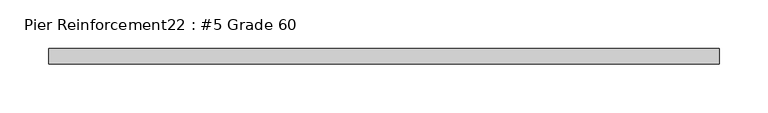
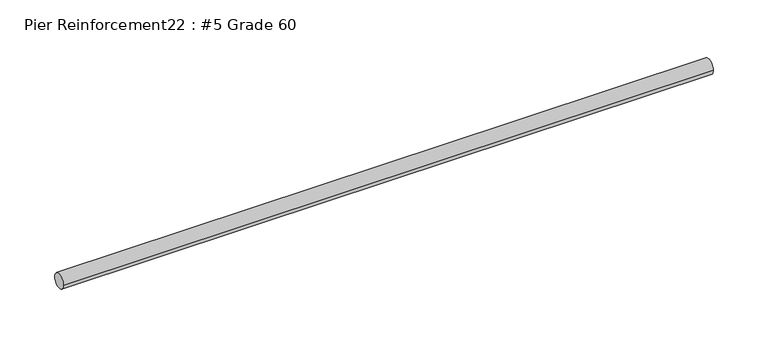
"""IFC4 building model written with IfcOpenShell, lengths in millimetres: proxy geometry, Pier Reinforcement22 : #5 Grade 60."""

from ifc_helpers import new_model, si_unit, point, frame, frame_2d, origin, place, context, project, spatial, circle_curve, trimmed, segment, composite_curve, outline, extrude, source, transform, mapped, element, save


def pier_reinforcement22_5_grade_60_586069a3(model_context):
    return source(origin(), model_context, "Body", "SweptSolid", [
        extrude(outline(composite_curve([segment(trimmed(circle_curve(frame_2d((-534096.6663841, -55.5625)), 7.9375), [point((-534088.7288841, -55.5625))], [point((-534104.6038841, -55.5625))], False, "CARTESIAN"), True, "CONTINUOUS"), segment(trimmed(circle_curve(frame_2d((-534096.6663841, -55.5625)), 7.9375), [point((-534104.6038841, -55.5625))], [point((-534088.7288841, -55.5625))], False, "CARTESIAN"), True, "CONTINUOUS")], self_intersect=False)), frame((589548.1922365, 0.0, 0.0), z_axis=(1.0, 0.0, 0.0), x_axis=(0.0, 1.0, 0.0)), (0.0, 0.0, 1.0), 685.8),
    ])


if __name__ == "__main__":
    model = new_model("IFC4")
    model_context = context("Model", 3, world=origin())
    ifc_project = project(units=[si_unit("LENGTHUNIT", "METRE", prefix="MILLI")], contexts=[model_context])
    site = spatial("IfcSite", under=ifc_project)
    building = spatial("IfcBuilding", under=site)
    placement = place(None, origin())
    pier_reinforcement22_5_grade_60_shape = pier_reinforcement22_5_grade_60_586069a3(model_context)
    element("IfcBuildingElementProxy", 1, Name="Pier Reinforcement22 : #5 Grade 60", ObjectType="Pier Reinforcement22 : #5 Grade 60", at=placement, inside=building, context=model_context, shape_type="MappedRepresentation", body=[
        mapped(pier_reinforcement22_5_grade_60_shape, transform((0.0, 0.0, 0.0), x_axis=(1.0, 0.0, 0.0), y_axis=(0.0, 1.0, 0.0), z_axis=(0.0, 0.0, 1.0))),
    ])
    save(model, "model.ifc")

# Revit data of these elements
# Element 1 (IfcBuildingElementProxy, "Pier Reinforcement22 : #5 Grade 60")
#   Materials on its faces: "#4 GR. 60 REINF. @ 16\" O.C. EW."
# Materials
#   "#4 GR. 60 REINF. @ 16\" O.C. EW.": class "Generic", colour RGB 84 83 81, transparency 0, Cost = 0
